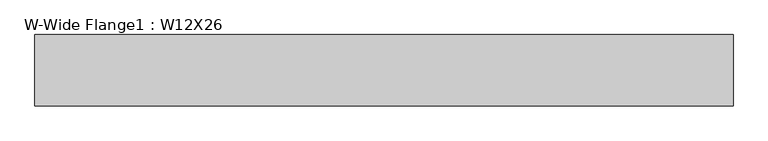
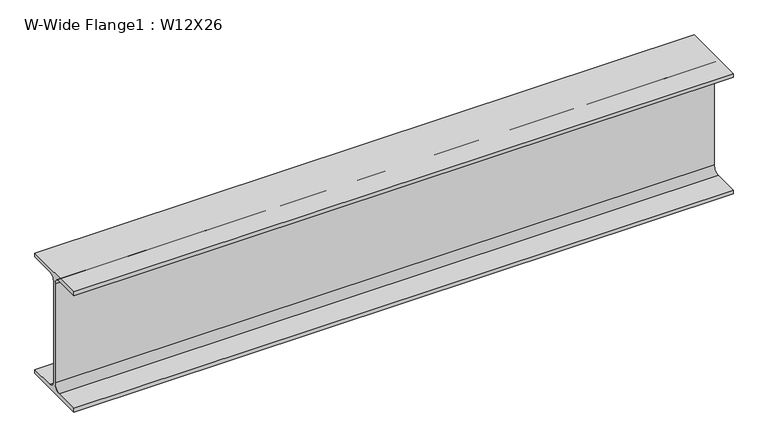
"""IFC4 building model written with IfcOpenShell, lengths in millimetres: beam geometry, W-Wide Flange1 : W12X26."""

from ifc_helpers import new_model, si_unit, point, frame, frame_2d, origin, place, context, project, spatial, polyline, circle_curve, trimmed, segment, composite_curve, outline, extrude, source, transform, mapped, element, save


def w_wide_flange1_w12x26_fc7dcb85(model_context):
    return source(origin(), model_context, "Body", "SweptSolid", [
        extrude(outline(composite_curve([segment(polyline([(82.423, -145.288), (82.423, -154.94), (-82.423, -154.94), (-82.423, -145.288), (-20.2565, -145.288)]), True, "CONTINUOUS"), segment(trimmed(circle_curve(frame_2d((-20.2565, -127.9525)), 17.3355), [point((-20.2565, -145.288))], [point((-2.921, -127.9525))], True, "CARTESIAN"), True, "CONTINUOUS"), segment(polyline([(-2.921, -127.9525), (-2.921, 127.9525)]), True, "CONTINUOUS"), segment(trimmed(circle_curve(frame_2d((-20.2565, 127.9525)), 17.3355), [point((-2.921, 127.9525))], [point((-20.2565, 145.288))], True, "CARTESIAN"), True, "CONTINUOUS"), segment(polyline([(-20.2565, 145.288), (-82.423, 145.288), (-82.423, 154.94), (82.423, 154.94), (82.423, 145.288), (20.2565, 145.288)]), True, "CONTINUOUS"), segment(trimmed(circle_curve(frame_2d((20.2565, 127.9525)), 17.3355), [point((20.2565, 145.288))], [point((2.921, 127.9525))], True, "CARTESIAN"), True, "CONTINUOUS"), segment(polyline([(2.921, 127.9525), (2.921, -127.9525)]), True, "CONTINUOUS"), segment(trimmed(circle_curve(frame_2d((20.2565, -127.9525)), 17.3355), [point((2.921, -127.9525))], [point((20.2565, -145.288))], True, "CARTESIAN"), True, "CONTINUOUS"), segment(polyline([(20.2565, -145.288), (82.423, -145.288)]), True, "CONTINUOUS")], self_intersect=False)), frame((-702.2871039, 0.0, 0.0), z_axis=(1.0, 0.0, 0.0), x_axis=(0.0, 1.0, 0.0)), (0.0, 0.0, 1.0), 1608.4551986),
    ])


if __name__ == "__main__":
    model = new_model("IFC4")
    model_context = context("Model", 3, world=origin())
    ifc_project = project(units=[si_unit("LENGTHUNIT", "METRE", prefix="MILLI")], contexts=[model_context])
    site = spatial("IfcSite", under=ifc_project)
    building = spatial("IfcBuilding", under=site)
    placement = place(None, origin())
    w_wide_flange1_w12x26_shape = w_wide_flange1_w12x26_fc7dcb85(model_context)
    element("IfcBeam", 1, ObjectType="W-Wide Flange1 : W12X26", at=placement, inside=building, context=model_context, shape_type="MappedRepresentation", body=[
        mapped(w_wide_flange1_w12x26_shape, transform((0.0, 0.0, 0.0), x_axis=(1.0, 0.0, 0.0), y_axis=(0.0, 1.0, 0.0), z_axis=(0.0, 0.0, 1.0))),
    ])
    save(model, "model.ifc")

# Revit data of these elements
# Type "W-Wide Flange1 : W12X26"
#   Assembly Code = "B10"
#   W = 26
#   Start Extension Calculation [instance default] = 10' - 0"
#   Start Extension [instance default] = -0' - 0 1/2"
#   End Extension Calculation [instance default] = 10' - 0"
#   End Extension [instance default] = -0' - 0 1/2"
#   Length [instance default] = 5' - 0"
#   bf = 0' - 6.49"
#   d = 1' - 0.2"
#   k = 0' - 1 1/16"
#   k2 = 0' - 0.6825"
#   tf = 0' - 0.38"
#   tw = 0' - 0.23"
#   A = 0.053125 SF
#   Structural Material [instance default] = Metal - Steel - ASTM A992
# Element 1 (IfcBeam, "W-Wide Flange1 : W12X26")
#   Materials on its faces: "Metal - Steel - ASTM A992"
# Materials
#   "Metal - Steel - ASTM A992": class "Metal", colour RGB 199 199 199, transparency 0
